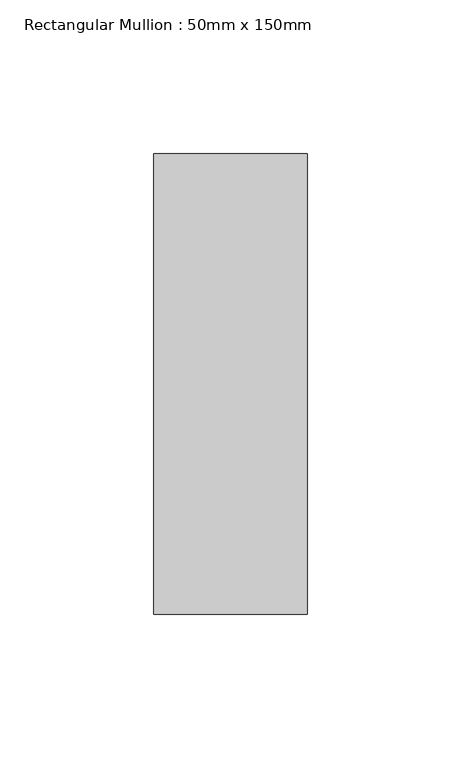
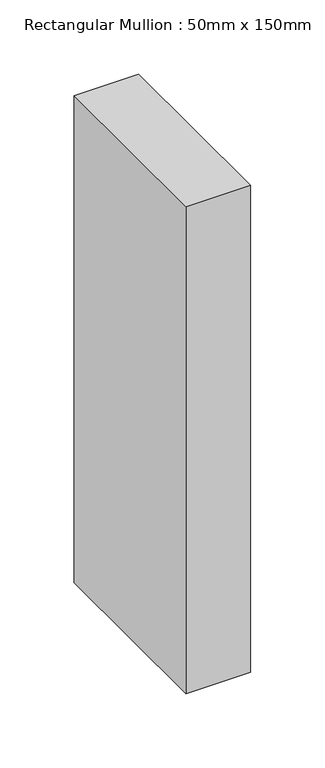
"""IFC4 building model written with IfcOpenShell, lengths in millimetres: member geometry, Rectangular Mullion : 50mm x 150mm."""

import ifcopenshell
import ifcopenshell.guid

model = None  # the IFC model being written
_history = None  # IfcOwnerHistory: only IFC2X3 demands one
_inside = {}  # id of a spatial element -> (the spatial element, [elements in it])
_under = {}  # id of a project, library or spatial element -> (it, [spatial elements below it])
_declared = {}  # id of a project -> (the project, [libraries it declares])
_typed = {}  # id of a type object -> (the type object, [elements of that type])
_made_of = {}  # id of a material, layer set ... -> (it, [elements and type objects made of it])


def new_model(schema):
    """Start an empty IFC model of exactly this schema.

    Asked for "IFC4X3", IfcOpenShell would pick the latest addendum, in which some entities
    have other attributes; the version numbers below select the first issue.
    IFC2X3 requires an IfcOwnerHistory on every rooted entity: one is made here for all.
    """
    global model, _history
    if schema == "IFC4X3":
        model = ifcopenshell.file(schema_version=(4, 3, 0, 0))
    else:
        model = ifcopenshell.file(schema=schema)
    _inside.clear()
    _under.clear()
    _declared.clear()
    _typed.clear()
    _made_of.clear()
    _history = None
    if model.schema == "IFC2X3":
        org = make("IfcOrganization", Name="unknown")
        user = make(
            "IfcPersonAndOrganization",
            ThePerson=make("IfcPerson", FamilyName="unknown"),
            TheOrganization=org,
        )
        app = make(
            "IfcApplication",
            ApplicationDeveloper=org,
            Version="unknown",
            ApplicationFullName="unknown",
            ApplicationIdentifier="unknown",
        )
        _history = make(
            "IfcOwnerHistory",
            OwningUser=user,
            OwningApplication=app,
            ChangeAction="ADDED",
            CreationDate=0,
        )
    return model


def make(cls, **values):
    """One entity of the class cls with the attributes given. An attribute that is None is left unset."""
    return model.create_entity(
        cls, **{name: value for name, value in values.items() if value is not None}
    )


def rooted(cls, **values):
    """An entity with a GlobalId (a new one), such as an element, a storey or a relation."""
    return make(cls, GlobalId=ifcopenshell.guid.new(), OwnerHistory=_history, **values)


def si_unit(unit_type, name, prefix=None):
    """IfcSIUnit, for example si_unit("LENGTHUNIT", "METRE", prefix="MILLI")."""
    return make("IfcSIUnit", UnitType=unit_type, Prefix=prefix, Name=name)


def assignment(units):
    """IfcUnitAssignment: the units of a project."""
    return None if units is None else make("IfcUnitAssignment", Units=units)


def point(xyz):
    """IfcCartesianPoint."""
    return None if xyz is None else make("IfcCartesianPoint", Coordinates=xyz)


def direction(xyz):
    """IfcDirection."""
    return None if xyz is None else make("IfcDirection", DirectionRatios=xyz)


def frame(location, z_axis=None, x_axis=None):
    """IfcAxis2Placement3D, a coordinate frame: its origin and axes. An axis left out is left unset."""
    return make(
        "IfcAxis2Placement3D",
        Location=point(location),
        Axis=direction(z_axis),
        RefDirection=direction(x_axis),
    )


def origin():
    """The frame at (0, 0, 0) with its axes left unset."""
    return frame((0.0, 0.0, 0.0))


def place(relative_to, where):
    """IfcLocalPlacement: puts the frame where relative to a parent placement (None: the world)."""
    return make(
        "IfcLocalPlacement", PlacementRelTo=relative_to, RelativePlacement=where
    )


def context(
    kind, dimensions, precision=None, world=None, true_north=None, identifier=None
):
    """IfcGeometricRepresentationContext, for example the 3D "Model" context."""
    return make(
        "IfcGeometricRepresentationContext",
        ContextIdentifier=identifier,
        ContextType=kind,
        CoordinateSpaceDimension=dimensions,
        Precision=precision,
        WorldCoordinateSystem=world,
        TrueNorth=true_north,
    )


def project(units=None, contexts=None):
    """IfcProject with its units and contexts."""
    return rooted(
        "IfcProject",
        Name="project",
        RepresentationContexts=contexts,
        UnitsInContext=assignment(units),
    )


def spatial(cls, under=None, at=None, **own):
    """A site, building, storey or space (cls), placed at a placement, below another one or the project."""
    s = rooted(cls, ObjectPlacement=at, **own)
    if under is not None:
        _under.setdefault(under.id(), (under, []))[1].append(s)
    return s


def polyline(points):
    """IfcPolyline through the points."""
    return make("IfcPolyline", Points=[point(p) for p in points])


def outline(outer, holes=None, kind="AREA"):
    """IfcArbitraryClosedProfileDef: a profile drawn as a closed curve; with holes, ...WithVoids."""
    if holes is None:
        return make("IfcArbitraryClosedProfileDef", ProfileType=kind, OuterCurve=outer)
    return make(
        "IfcArbitraryProfileDefWithVoids",
        ProfileType=kind,
        OuterCurve=outer,
        InnerCurves=holes,
    )


def extrude(swept, where, along, depth):
    """IfcExtrudedAreaSolid: the profile swept, set in the frame where, extruded along a direction by depth."""
    return make(
        "IfcExtrudedAreaSolid",
        SweptArea=swept,
        Position=where,
        ExtrudedDirection=direction(along),
        Depth=depth,
    )


def shape(context_of_items, identifier, shape_type, items):
    """IfcShapeRepresentation: the items that make up one representation, for example the "Body"."""
    return make(
        "IfcShapeRepresentation",
        ContextOfItems=context_of_items,
        RepresentationIdentifier=identifier,
        RepresentationType=shape_type,
        Items=items,
    )


def source(mapping_origin, context_of_items, identifier, shape_type, items):
    """IfcRepresentationMap: a shape defined once, which mapped items show again and again."""
    return make(
        "IfcRepresentationMap",
        MappingOrigin=mapping_origin,
        MappedRepresentation=shape(context_of_items, identifier, shape_type, items),
    )


def transform(
    local_origin,
    x_axis=None,
    y_axis=None,
    z_axis=None,
    scale=None,
    scale2=None,
    scale3=None,
    uniform=True,
):
    """IfcCartesianTransformationOperator3D, or its non-uniform kind. x_axis, y_axis, z_axis: its Axis1, 2, 3."""
    if uniform:
        return make(
            "IfcCartesianTransformationOperator3D",
            Axis1=direction(x_axis),
            Axis2=direction(y_axis),
            LocalOrigin=point(local_origin),
            Scale=scale,
            Axis3=direction(z_axis),
        )
    return make(
        "IfcCartesianTransformationOperator3DnonUniform",
        Axis1=direction(x_axis),
        Axis2=direction(y_axis),
        LocalOrigin=point(local_origin),
        Scale=scale,
        Axis3=direction(z_axis),
        Scale2=scale2,
        Scale3=scale3,
    )


def mapped(mapping_source, mapping_target):
    """IfcMappedItem: shows the shape of a source again, moved by a transform."""
    return make(
        "IfcMappedItem", MappingSource=mapping_source, MappingTarget=mapping_target
    )


def made_of(thing, what):
    """Note that an element or type object is made of a material, layer set ...; save() writes the relation."""
    if what is not None:
        _made_of.setdefault(what.id(), (what, []))[1].append(thing)
    return thing


def element(
    cls,
    number,
    at=None,
    inside=None,
    cuts=None,
    type_object=None,
    material=None,
    context=None,
    identifier="Body",
    shape_type=None,
    held_by="IfcProductDefinitionShape",
    body=None,
    shapes=None,
    **own,
):
    """One element of the class cls, such as IfcWall. Its Tag is "e" and its number.

    at: its placement. inside: the storey or other place that contains it. cuts: it is an
    opening in that element (IfcRelVoidsElement). A single representation is given by context,
    identifier, shape_type and body (its items); several are given by shapes. held_by: the class
    of the entity that holds the representations. save() writes the other relations.
    """
    e = rooted(cls, Tag="e%d" % number, ObjectPlacement=at, **own)
    if body is not None:
        shapes = [shape(context, identifier, shape_type, body)]
    if shapes is not None:
        e.Representation = make(held_by, Representations=shapes)
    if inside is not None:
        _inside.setdefault(inside.id(), (inside, []))[1].append(e)
    if cuts is not None:
        rooted(
            "IfcRelVoidsElement", RelatingBuildingElement=cuts, RelatedOpeningElement=e
        )
    if type_object is not None:
        _typed.setdefault(type_object.id(), (type_object, []))[1].append(e)
    return made_of(e, material)


def aggregate(whole, parts):
    """IfcRelAggregates: a whole, such as a stair, and the parts it consists of."""
    return rooted("IfcRelAggregates", RelatingObject=whole, RelatedObjects=parts)


def save(model, path):
    """Write the relations noted so far, then the file.

    IfcRelAggregates (storeys below a building ...), IfcRelContainedInSpatialStructure (elements
    in a storey), IfcRelDefinesByType, IfcRelAssociatesMaterial and IfcRelDeclares: one each for
    every whole, place, type object, material and project.
    """
    for whole, parts in _under.values():
        aggregate(whole, parts)
    for where, things in _inside.values():
        rooted(
            "IfcRelContainedInSpatialStructure",
            RelatedElements=things,
            RelatingStructure=where,
        )
    for kind, things in _typed.values():
        rooted("IfcRelDefinesByType", RelatedObjects=things, RelatingType=kind)
    for what, things in _made_of.values():
        rooted("IfcRelAssociatesMaterial", RelatedObjects=things, RelatingMaterial=what)
    for by, libraries in _declared.values():
        rooted("IfcRelDeclares", RelatingContext=by, RelatedDefinitions=libraries)
    model.write(path)


def rectangular_mullion_50mm_x_150mm_07b0a205(model_context):
    return source(origin(), model_context, "Body", "SweptSolid", [
        extrude(outline(polyline([(25.0, 75.0), (25.0, -75.0), (-25.0, -75.0), (-25.0, 75.0), (25.0, 75.0)])), frame((0.0, 0.0, -398.8777657), z_axis=(0.0, 0.0, 1.0), x_axis=(1.0, 0.0, 0.0)), (0.0, 0.0, 1.0), 398.8777657),
    ])


if __name__ == "__main__":
    model = new_model("IFC4")
    model_context = context("Model", 3, world=origin())
    ifc_project = project(units=[si_unit("LENGTHUNIT", "METRE", prefix="MILLI")], contexts=[model_context])
    site = spatial("IfcSite", under=ifc_project)
    building = spatial("IfcBuilding", under=site)
    placement = place(None, origin())
    rectangular_mullion_50mm_x_150mm_shape = rectangular_mullion_50mm_x_150mm_07b0a205(model_context)
    element("IfcMember", 1, ObjectType="Rectangular Mullion : 50mm x 150mm", at=placement, inside=building, context=model_context, shape_type="MappedRepresentation", body=[
        mapped(rectangular_mullion_50mm_x_150mm_shape, transform((0.0, 0.0, 0.0), x_axis=(1.0, 0.0, 0.0), y_axis=(0.0, 1.0, 0.0), z_axis=(0.0, 0.0, 1.0))),
    ])
    save(model, "model.ifc")

# Revit data of these elements
# Type "Rectangular Mullion : 50mm x 150mm"
#   built-in parameter 1007304 = 0.492126 (stored number, unit not read)
#   built-in parameter 1007301 = 0.082021 (stored number, unit not read)
#   built-in parameter 1007300 = 0.082021 (stored number, unit not read)
# Element 1 (IfcMember, "Rectangular Mullion : 50mm x 150mm")
#   Materials on its faces: "Aluminum"
# Materials
#   "Aluminum": class "Metal", colour RGB 244 244 244, transparency 0, Description = "Aluminum 6061", Cost = 0
